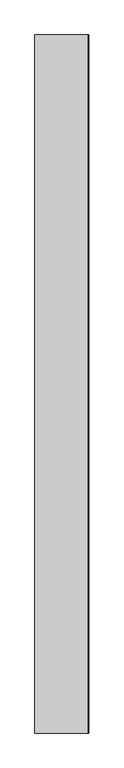
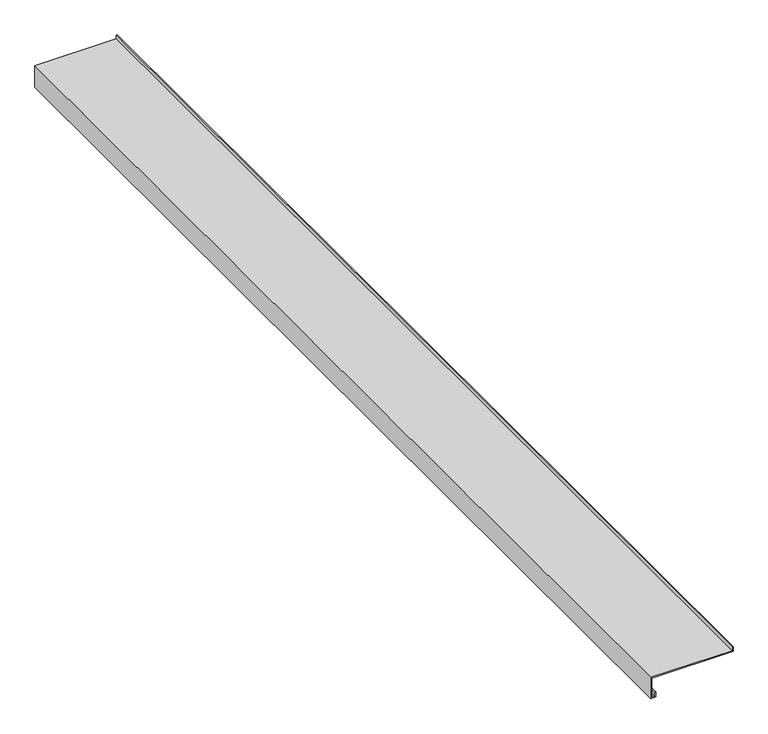
"""IFC4 building model written with IfcOpenShell, lengths in millimetres: proxy geometry, Flashing026 14415 : Flashing026 14415."""

from ifc_helpers import new_model, si_unit, frame, origin, place, context, project, spatial, polyline, outline, extrude, source, transform, mapped, element, save


def generic_models_3ad6fd26(model_context):
    return source(origin(), model_context, "Body", "SweptSolid", [
        extrude(outline(polyline([(36566.1804687, -1997.9650879), (36558.9851563, -1997.9650879), (36558.9851563, -2150.7495117), (36516.8054688, -2150.7495117), (36516.8054688, -2140.6896973), (36527.3601562, -2140.6896973), (36527.3601562, -2142.6896973), (36518.8054687, -2142.6896973), (36518.8054687, -2148.7495117), (36556.9851562, -2148.7495117), (36556.9851562, -1995.9650879), (36566.1804687, -1995.9650879), (36566.1804687, -1997.9650879)])), frame((0.0, 998.1570053, 0.0), z_axis=(0.0, 1.0, 0.0), x_axis=(0.0, 0.0, 1.0)), (0.0, 0.0, 1.0), 2000.0),
    ])


if __name__ == "__main__":
    model = new_model("IFC4")
    model_context = context("Model", 3, world=origin())
    ifc_project = project(units=[si_unit("LENGTHUNIT", "METRE", prefix="MILLI")], contexts=[model_context])
    site = spatial("IfcSite", under=ifc_project)
    building = spatial("IfcBuilding", under=site)
    placement = place(None, origin())
    generic_models_shape = generic_models_3ad6fd26(model_context)
    element("IfcBuildingElementProxy", 1, Name="Flashing026 14415 : Flashing026 14415", ObjectType="Flashing026 14415 : Flashing026 14415", at=placement, inside=building, context=model_context, shape_type="MappedRepresentation", body=[
        mapped(generic_models_shape, transform((0.0, 0.0, 0.0), x_axis=(1.0, 0.0, 0.0), y_axis=(0.0, 1.0, 0.0), z_axis=(0.0, 0.0, 1.0))),
    ])
    save(model, "model.ifc")

# Revit data of these elements
# Type "Flashing026 14415 : Flashing026 14415"
#   NameOverride = "Flashing026"
# Element 1 (IfcBuildingElementProxy, "Flashing026 14415 : Flashing026 14415")
#   Materials on its faces: "16GA. COPPER BRAKE METAL FLASHING"
# Materials
#   "16GA. COPPER BRAKE METAL FLASHING": class "Unassigned", colour RGB 128 128 128, transparency 0
